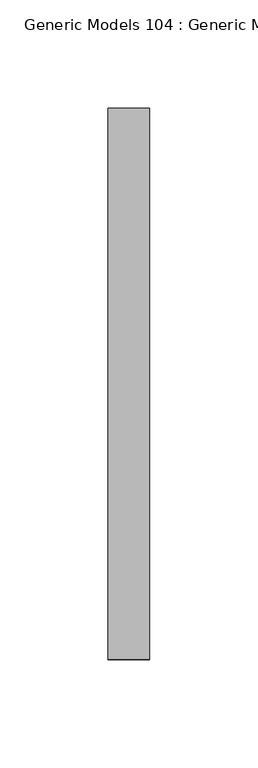
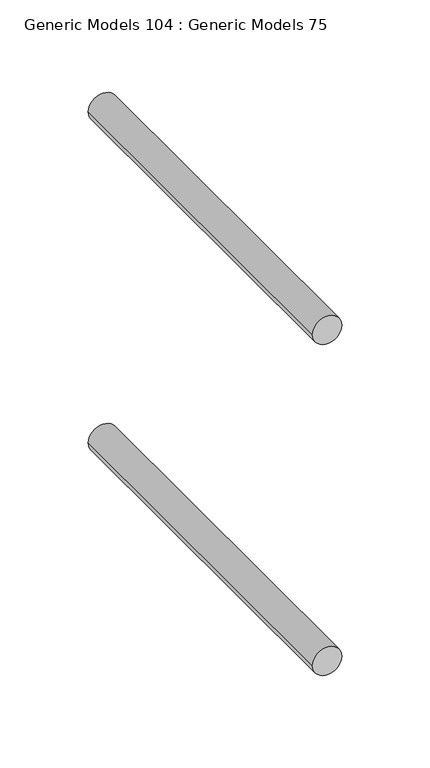
"""IFC4 building model written with IfcOpenShell, lengths in millimetres: proxy geometry, Generic Models 104 : Generic Models 75."""

from ifc_helpers import new_model, si_unit, point, frame, frame_2d, origin, place, context, project, spatial, circle_curve, trimmed, segment, composite_curve, outline, extrude, source, transform, mapped, element, save


def generic_models_104_generic_models_75_128766d0(model_context):
    return source(origin(), model_context, "Body", "SweptSolid", [
        extrude(outline(composite_curve([segment(trimmed(circle_curve(frame_2d((269062.2, 31975.4096032)), 9.525), [point((269062.2, 31965.8846032))], [point((269062.2, 31984.9346032))], False, "CARTESIAN"), True, "CONTINUOUS"), segment(trimmed(circle_curve(frame_2d((269062.2, 31975.4096032)), 9.525), [point((269062.2, 31984.9346032))], [point((269062.2, 31965.8846032))], False, "CARTESIAN"), True, "CONTINUOUS")], self_intersect=False)), frame((0.0, 30647.3406612, 0.0), z_axis=(0.0, 1.0, 0.0), x_axis=(0.0, 0.0, 1.0)), (0.0, 0.0, 1.0), 254.0),
        extrude(outline(composite_curve([segment(trimmed(circle_curve(frame_2d((268833.6, 31975.4096032)), 9.525), [point((268833.6, 31965.8846032))], [point((268833.6, 31984.9346032))], False, "CARTESIAN"), True, "CONTINUOUS"), segment(trimmed(circle_curve(frame_2d((268833.6, 31975.4096032)), 9.525), [point((268833.6, 31984.9346032))], [point((268833.6, 31965.8846032))], False, "CARTESIAN"), True, "CONTINUOUS")], self_intersect=False)), frame((0.0, 30647.3406612, 0.0), z_axis=(0.0, 1.0, 0.0), x_axis=(0.0, 0.0, 1.0)), (0.0, 0.0, 1.0), 254.0),
    ])


if __name__ == "__main__":
    model = new_model("IFC4")
    model_context = context("Model", 3, world=origin())
    ifc_project = project(units=[si_unit("LENGTHUNIT", "METRE", prefix="MILLI")], contexts=[model_context])
    site = spatial("IfcSite", under=ifc_project)
    building = spatial("IfcBuilding", under=site)
    placement = place(None, origin())
    generic_models_104_generic_models_75_shape = generic_models_104_generic_models_75_128766d0(model_context)
    element("IfcBuildingElementProxy", 1, Name="Generic Models 104 : Generic Models 75", ObjectType="Generic Models 104 : Generic Models 75", at=placement, inside=building, context=model_context, shape_type="MappedRepresentation", body=[
        mapped(generic_models_104_generic_models_75_shape, transform((0.0, 0.0, 0.0), x_axis=(1.0, 0.0, 0.0), y_axis=(0.0, 1.0, 0.0), z_axis=(0.0, 0.0, 1.0))),
    ])
    save(model, "model.ifc")
